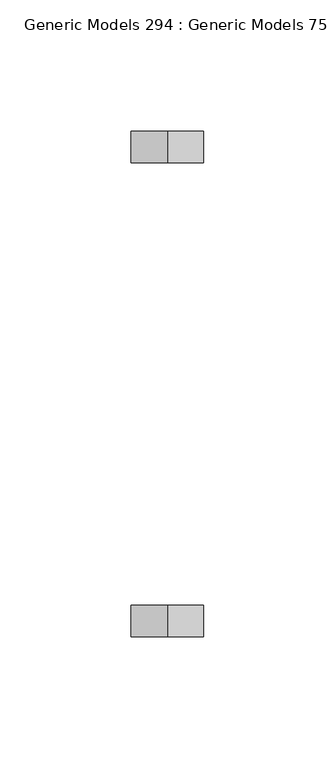
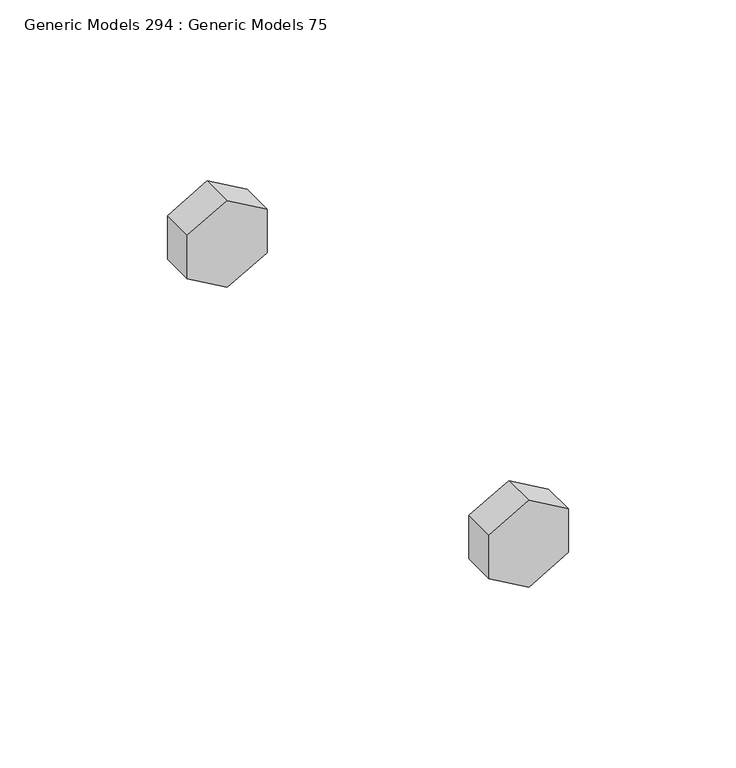
"""IFC4 building model written with IfcOpenShell, lengths in millimetres: proxy geometry, Generic Models 294 : Generic Models 75."""

from ifc_helpers import new_model, si_unit, frame, origin, place, context, project, spatial, polyline, outline, extrude, source, transform, mapped, element, save


def generic_models_294_generic_models_75_af934234(model_context):
    return source(origin(), model_context, "Body", "SweptSolid", [
        extrude(outline(polyline([(268765.3182867, 31975.9942029), (268749.4817133, 31975.9942029), (268741.5634265, 31989.7090778), (268749.4817133, 32003.4239528), (268765.3182867, 32003.4239528), (268773.2365735, 31989.7090778), (268765.3182867, 31975.9942029)])), frame((0.0, 35373.9582942, 0.0), z_axis=(0.0, 1.0, 0.0), x_axis=(0.0, 0.0, 1.0)), (0.0, 0.0, 1.0), 11.90625),
        extrude(outline(polyline([(268765.3182867, 31975.9942029), (268749.4817133, 31975.9942029), (268741.5634265, 31989.7090778), (268749.4817133, 32003.4239528), (268765.3182867, 32003.4239528), (268773.2365735, 31989.7090778), (268765.3182867, 31975.9942029)])), frame((0.0, 35193.7770442, 0.0), z_axis=(0.0, 1.0, 0.0), x_axis=(0.0, 0.0, 1.0)), (0.0, 0.0, 1.0), 11.90625),
    ])


if __name__ == "__main__":
    model = new_model("IFC4")
    model_context = context("Model", 3, world=origin())
    ifc_project = project(units=[si_unit("LENGTHUNIT", "METRE", prefix="MILLI")], contexts=[model_context])
    site = spatial("IfcSite", under=ifc_project)
    building = spatial("IfcBuilding", under=site)
    placement = place(None, origin())
    generic_models_294_generic_models_75_shape = generic_models_294_generic_models_75_af934234(model_context)
    element("IfcBuildingElementProxy", 1, Name="Generic Models 294 : Generic Models 75", ObjectType="Generic Models 294 : Generic Models 75", at=placement, inside=building, context=model_context, shape_type="MappedRepresentation", body=[
        mapped(generic_models_294_generic_models_75_shape, transform((0.0, 0.0, 0.0), x_axis=(1.0, 0.0, 0.0), y_axis=(0.0, 1.0, 0.0), z_axis=(0.0, 0.0, 1.0))),
    ])
    save(model, "model.ifc")

# Revit data of these elements
# Element 1 (IfcBuildingElementProxy, "Generic Models 294 : Generic Models 75")
#   Materials on its faces: "3/4\" GALV. THRU BOLTS"
# Materials
#   "3/4\" GALV. THRU BOLTS": class "Generic", colour RGB 105 69 171, transparency 0, Cost = 0
